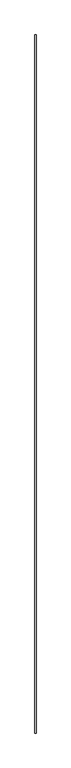
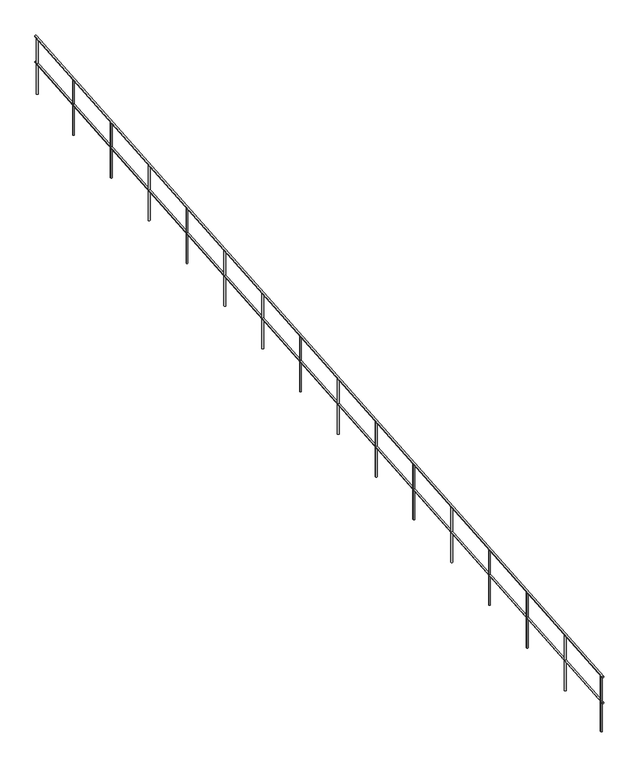
"""IFC4 building model written with IfcOpenShell, lengths in millimetres: railing geometry."""

from ifc_helpers import new_model, si_unit, frame, origin, place, context, project, spatial, ellipse_curve, source, transform, mapped, element, save
from ifc_brep_helpers import plane_surface, cylinder_surface, advanced_brep


def railing_917cd56d(model_context):
    return source(origin(), model_context, "Body", "AdvancedBrep", [
        advanced_brep(
        [(-7531.0, 39498.9598199, -615.0519932), (-7501.0, 39498.9598199, -615.0519932), (-7531.0, 57498.9598198, 884.9480068), (-7501.0, 57498.9598198, 884.9480068)],
        [
            (0, 1, ellipse_curve(frame((-7516.0, 39498.9598199, -615.0519932), z_axis=(0.0, -1.0, 0.0), x_axis=(0.0, 0.0, -0.9999999999999999)), 15.0519932, 15.0)),
            (1, 0, ellipse_curve(frame((-7516.0, 39498.9598199, -615.0519932), z_axis=(0.0, -1.0, 0.0), x_axis=(0.0, 0.0, -0.9999999999999999)), 15.0519932, 15.0)),
            (2, 3, ellipse_curve(frame((-7516.0, 57498.9598198, 884.9480068), z_axis=(0.0, 1.0, 0.0), x_axis=(0.0, 0.0, -0.9999999999999999)), 15.0519932, 15.0)),
            (3, 2, ellipse_curve(frame((-7516.0, 57498.9598198, 884.9480068), z_axis=(0.0, 1.0, 0.0), x_axis=(0.0, 0.0, -0.9999999999999999)), 15.0519932, 15.0)),
            (0, 2),
            (3, 1),
        ],
        [
            plane_surface(frame((-7516.0, 39498.9598199, -600.0), z_axis=(0.0, -1.0, 0.0), x_axis=(0.0, 0.0, 1.0))),
            plane_surface(frame((-7516.0, 57498.9598198, 900.0), z_axis=(0.0, 1.0, 0.0), x_axis=(0.0, 0.0, 1.0))),
            cylinder_surface(frame((-7516.0, 39500.2055021, -614.9481864), z_axis=(0.0, -0.9965457582448797, -0.08304547985373997), x_axis=(1.0, 0.0, 0.0)), 15.0),
        ],
        [
            (0, [[1, 2]]),
            (1, [[3, 4]]),
            (2, [[-1, 5, -4, 6]]),
            (2, [[-2, -6, -3, -5]]),
        ],
    ),
        advanced_brep(
        [(-7531.0, 39498.9598199, -115.0519932), (-7501.0, 39498.9598199, -115.0519932), (-7531.0, 57498.9598198, 1384.9480068), (-7501.0, 57498.9598198, 1384.9480068)],
        [
            (0, 1, ellipse_curve(frame((-7516.0, 39498.9598199, -115.0519932), z_axis=(0.0, -1.0, 0.0), x_axis=(0.0, 0.0, -0.9999999999999999)), 15.0519932, 15.0)),
            (1, 0, ellipse_curve(frame((-7516.0, 39498.9598199, -115.0519932), z_axis=(0.0, -1.0, 0.0), x_axis=(0.0, 0.0, -0.9999999999999999)), 15.0519932, 15.0)),
            (2, 3, ellipse_curve(frame((-7516.0, 57498.9598198, 1384.9480068), z_axis=(0.0, 1.0, 0.0), x_axis=(0.0, 0.0, -0.9999999999999999)), 15.0519932, 15.0)),
            (3, 2, ellipse_curve(frame((-7516.0, 57498.9598198, 1384.9480068), z_axis=(0.0, 1.0, 0.0), x_axis=(0.0, 0.0, -0.9999999999999999)), 15.0519932, 15.0)),
            (0, 2),
            (3, 1),
        ],
        [
            plane_surface(frame((-7516.0, 39498.9598199, -100.0), z_axis=(0.0, -1.0, 0.0), x_axis=(0.0, 0.0, 1.0))),
            plane_surface(frame((-7516.0, 57498.9598198, 1400.0), z_axis=(0.0, 1.0, 0.0), x_axis=(0.0, 0.0, 1.0))),
            cylinder_surface(frame((-7516.0, 39500.2055021, -114.9481864), z_axis=(0.0, -0.9965457582448797, -0.08304547985373997), x_axis=(1.0, 0.0, 0.0)), 15.0),
        ],
        [
            (0, [[1, 2]]),
            (1, [[3, 4]]),
            (2, [[-1, 5, -4, 6]]),
            (2, [[-2, -6, -3, -5]]),
        ],
    ),
        advanced_brep(
        [(-7501.0, 56298.9598199, 1269.8960136), (-7501.0, 56298.9598199, 200.0), (-7531.0, 56298.9598199, 200.0), (-7531.0, 56298.9598199, 1269.8960136)],
        [
            (0, 1),
            (1, 2, ellipse_curve(frame((-7516.0, 56298.9598199, 200.0), z_axis=(0.0, -0.08304547985373996, 0.9965457582448797), x_axis=(0.0, 0.9965457582448798, 0.08304547985373881)), 15.0519932, 15.0)),
            (2, 3),
            (3, 0, ellipse_curve(frame((-7516.0, 56298.9598199, 1269.8960136), z_axis=(0.0, 0.083045479853741, -0.9965457582448796), x_axis=(0.0, 0.9965457582448797, 0.08304547985374044)), 15.0519932, 15.0)),
            (0, 3, ellipse_curve(frame((-7516.0, 56298.9598199, 1269.8960136), z_axis=(0.0, 0.083045479853741, -0.9965457582448796), x_axis=(0.0, 0.9965457582448797, 0.08304547985374044)), 15.0519932, 15.0)),
            (2, 1, ellipse_curve(frame((-7516.0, 56298.9598199, 200.0), z_axis=(0.0, -0.08304547985373996, 0.9965457582448797), x_axis=(0.0, 0.9965457582448798, 0.08304547985373881)), 15.0519932, 15.0)),
        ],
        [
            cylinder_surface(frame((-7516.0, 56298.9598199, 100.0), z_axis=(0.0, 0.0, 1.0), x_axis=(-1.0, 0.0, 0.0)), 15.0),
            plane_surface(frame((-7541.0, 56323.9598199, 1271.9793469), z_axis=(0.0, -0.083045479853741, 0.9965457582448796), x_axis=(1.0, 0.0, 0.0))),
            plane_surface(frame((-7541.0, 56273.9598199, 197.9166667), z_axis=(0.0, 0.08304547985373996, -0.9965457582448797), x_axis=(1.0, 0.0, 0.0))),
        ],
        [
            (0, [[1, 2, 3, 4]]),
            (0, [[-1, 5, -3, 6]]),
            (1, [[-4, -5]]),
            (2, [[-2, -6]]),
        ],
    ),
        advanced_brep(
        [(-7501.0, 55098.9598199, 1169.8960136), (-7501.0, 55098.9598199, 100.0), (-7531.0, 55098.9598199, 100.0), (-7531.0, 55098.9598199, 1169.8960136)],
        [
            (0, 1),
            (1, 2, ellipse_curve(frame((-7516.0, 55098.9598199, 100.0), z_axis=(0.0, -0.08304547985373996, 0.9965457582448797), x_axis=(0.0, 0.9965457582448798, 0.08304547985373881)), 15.0519932, 15.0)),
            (2, 3),
            (3, 0, ellipse_curve(frame((-7516.0, 55098.9598199, 1169.8960136), z_axis=(0.0, 0.083045479853741, -0.9965457582448796), x_axis=(0.0, 0.9965457582448797, 0.08304547985374044)), 15.0519932, 15.0)),
            (0, 3, ellipse_curve(frame((-7516.0, 55098.9598199, 1169.8960136), z_axis=(0.0, 0.083045479853741, -0.9965457582448796), x_axis=(0.0, 0.9965457582448797, 0.08304547985374044)), 15.0519932, 15.0)),
            (2, 1, ellipse_curve(frame((-7516.0, 55098.9598199, 100.0), z_axis=(0.0, -0.08304547985373996, 0.9965457582448797), x_axis=(0.0, 0.9965457582448798, 0.08304547985373881)), 15.0519932, 15.0)),
        ],
        [
            cylinder_surface(frame((-7516.0, 55098.9598199, 0.0), z_axis=(0.0, 0.0, 1.0), x_axis=(-1.0, 0.0, 0.0)), 15.0),
            plane_surface(frame((-7541.0, 55123.9598199, 1171.9793469), z_axis=(0.0, -0.083045479853741, 0.9965457582448796), x_axis=(1.0, 0.0, 0.0))),
            plane_surface(frame((-7541.0, 55073.9598199, 97.9166667), z_axis=(0.0, 0.08304547985373996, -0.9965457582448797), x_axis=(1.0, 0.0, 0.0))),
        ],
        [
            (0, [[1, 2, 3, 4]]),
            (0, [[-1, 5, -3, 6]]),
            (1, [[-4, -5]]),
            (2, [[-2, -6]]),
        ],
    ),
        advanced_brep(
        [(-7501.0, 53898.9598199, 1069.8960136), (-7501.0, 53898.9598199, 0.0), (-7531.0, 53898.9598199, 0.0), (-7531.0, 53898.9598199, 1069.8960136)],
        [
            (0, 1),
            (1, 2, ellipse_curve(frame((-7516.0, 53898.9598199, 0.0), z_axis=(0.0, -0.08304547985373996, 0.9965457582448797), x_axis=(0.0, 0.9965457582448798, 0.08304547985373881)), 15.0519932, 15.0)),
            (2, 3),
            (3, 0, ellipse_curve(frame((-7516.0, 53898.9598199, 1069.8960136), z_axis=(0.0, 0.083045479853741, -0.9965457582448796), x_axis=(0.0, 0.9965457582448797, 0.08304547985374044)), 15.0519932, 15.0)),
            (0, 3, ellipse_curve(frame((-7516.0, 53898.9598199, 1069.8960136), z_axis=(0.0, 0.083045479853741, -0.9965457582448796), x_axis=(0.0, 0.9965457582448797, 0.08304547985374044)), 15.0519932, 15.0)),
            (2, 1, ellipse_curve(frame((-7516.0, 53898.9598199, 0.0), z_axis=(0.0, -0.08304547985373996, 0.9965457582448797), x_axis=(0.0, 0.9965457582448798, 0.08304547985373881)), 15.0519932, 15.0)),
        ],
        [
            cylinder_surface(frame((-7516.0, 53898.9598199, -100.0), z_axis=(0.0, 0.0, 1.0), x_axis=(-1.0, 0.0, 0.0)), 15.0),
            plane_surface(frame((-7541.0, 53923.9598199, 1071.9793469), z_axis=(0.0, -0.083045479853741, 0.9965457582448796), x_axis=(1.0, 0.0, 0.0))),
            plane_surface(frame((-7541.0, 53873.9598199, -2.0833333), z_axis=(0.0, 0.08304547985373996, -0.9965457582448797), x_axis=(1.0, 0.0, 0.0))),
        ],
        [
            (0, [[1, 2, 3, 4]]),
            (0, [[-1, 5, -3, 6]]),
            (1, [[-4, -5]]),
            (2, [[-2, -6]]),
        ],
    ),
        advanced_brep(
        [(-7501.0, 52698.9598199, 969.8960136), (-7501.0, 52698.9598199, -100.0), (-7531.0, 52698.9598199, -100.0), (-7531.0, 52698.9598199, 969.8960136)],
        [
            (0, 1),
            (1, 2, ellipse_curve(frame((-7516.0, 52698.9598199, -100.0), z_axis=(0.0, -0.08304547985373996, 0.9965457582448797), x_axis=(0.0, 0.9965457582448798, 0.08304547985373881)), 15.0519932, 15.0)),
            (2, 3),
            (3, 0, ellipse_curve(frame((-7516.0, 52698.9598199, 969.8960136), z_axis=(0.0, 0.083045479853741, -0.9965457582448796), x_axis=(0.0, 0.9965457582448797, 0.08304547985374044)), 15.0519932, 15.0)),
            (0, 3, ellipse_curve(frame((-7516.0, 52698.9598199, 969.8960136), z_axis=(0.0, 0.083045479853741, -0.9965457582448796), x_axis=(0.0, 0.9965457582448797, 0.08304547985374044)), 15.0519932, 15.0)),
            (2, 1, ellipse_curve(frame((-7516.0, 52698.9598199, -100.0), z_axis=(0.0, -0.08304547985373996, 0.9965457582448797), x_axis=(0.0, 0.9965457582448798, 0.08304547985373881)), 15.0519932, 15.0)),
        ],
        [
            cylinder_surface(frame((-7516.0, 52698.9598199, -200.0), z_axis=(0.0, 0.0, 1.0), x_axis=(-1.0, 0.0, 0.0)), 15.0),
            plane_surface(frame((-7541.0, 52723.9598199, 971.9793469), z_axis=(0.0, -0.083045479853741, 0.9965457582448796), x_axis=(1.0, 0.0, 0.0))),
            plane_surface(frame((-7541.0, 52673.9598199, -102.0833333), z_axis=(0.0, 0.08304547985373996, -0.9965457582448797), x_axis=(1.0, 0.0, 0.0))),
        ],
        [
            (0, [[1, 2, 3, 4]]),
            (0, [[-1, 5, -3, 6]]),
            (1, [[-4, -5]]),
            (2, [[-2, -6]]),
        ],
    ),
        advanced_brep(
        [(-7501.0, 51498.9598199, 869.8960136), (-7501.0, 51498.9598199, -200.0), (-7531.0, 51498.9598199, -200.0), (-7531.0, 51498.9598199, 869.8960136)],
        [
            (0, 1),
            (1, 2, ellipse_curve(frame((-7516.0, 51498.9598199, -200.0), z_axis=(0.0, -0.08304547985373996, 0.9965457582448797), x_axis=(0.0, 0.9965457582448798, 0.08304547985373881)), 15.0519932, 15.0)),
            (2, 3),
            (3, 0, ellipse_curve(frame((-7516.0, 51498.9598199, 869.8960136), z_axis=(0.0, 0.083045479853741, -0.9965457582448796), x_axis=(0.0, 0.9965457582448797, 0.08304547985374044)), 15.0519932, 15.0)),
            (0, 3, ellipse_curve(frame((-7516.0, 51498.9598199, 869.8960136), z_axis=(0.0, 0.083045479853741, -0.9965457582448796), x_axis=(0.0, 0.9965457582448797, 0.08304547985374044)), 15.0519932, 15.0)),
            (2, 1, ellipse_curve(frame((-7516.0, 51498.9598199, -200.0), z_axis=(0.0, -0.08304547985373996, 0.9965457582448797), x_axis=(0.0, 0.9965457582448798, 0.08304547985373881)), 15.0519932, 15.0)),
        ],
        [
            cylinder_surface(frame((-7516.0, 51498.9598199, -300.0), z_axis=(0.0, 0.0, 1.0), x_axis=(-1.0, 0.0, 0.0)), 15.0),
            plane_surface(frame((-7541.0, 51523.9598199, 871.9793469), z_axis=(0.0, -0.083045479853741, 0.9965457582448796), x_axis=(1.0, 0.0, 0.0))),
            plane_surface(frame((-7541.0, 51473.9598199, -202.0833333), z_axis=(0.0, 0.08304547985373996, -0.9965457582448797), x_axis=(1.0, 0.0, 0.0))),
        ],
        [
            (0, [[1, 2, 3, 4]]),
            (0, [[-1, 5, -3, 6]]),
            (1, [[-4, -5]]),
            (2, [[-2, -6]]),
        ],
    ),
        advanced_brep(
        [(-7501.0, 50298.9598199, 769.8960136), (-7501.0, 50298.9598199, -300.0), (-7531.0, 50298.9598199, -300.0), (-7531.0, 50298.9598199, 769.8960136)],
        [
            (0, 1),
            (1, 2, ellipse_curve(frame((-7516.0, 50298.9598199, -300.0), z_axis=(0.0, -0.08304547985373996, 0.9965457582448797), x_axis=(0.0, 0.9965457582448798, 0.08304547985373881)), 15.0519932, 15.0)),
            (2, 3),
            (3, 0, ellipse_curve(frame((-7516.0, 50298.9598199, 769.8960136), z_axis=(0.0, 0.083045479853741, -0.9965457582448796), x_axis=(0.0, 0.9965457582448797, 0.08304547985374044)), 15.0519932, 15.0)),
            (0, 3, ellipse_curve(frame((-7516.0, 50298.9598199, 769.8960136), z_axis=(0.0, 0.083045479853741, -0.9965457582448796), x_axis=(0.0, 0.9965457582448797, 0.08304547985374044)), 15.0519932, 15.0)),
            (2, 1, ellipse_curve(frame((-7516.0, 50298.9598199, -300.0), z_axis=(0.0, -0.08304547985373996, 0.9965457582448797), x_axis=(0.0, 0.9965457582448798, 0.08304547985373881)), 15.0519932, 15.0)),
        ],
        [
            cylinder_surface(frame((-7516.0, 50298.9598199, -400.0), z_axis=(0.0, 0.0, 1.0), x_axis=(-1.0, 0.0, 0.0)), 15.0),
            plane_surface(frame((-7541.0, 50323.9598199, 771.9793469), z_axis=(0.0, -0.083045479853741, 0.9965457582448796), x_axis=(1.0, 0.0, 0.0))),
            plane_surface(frame((-7541.0, 50273.9598199, -302.0833333), z_axis=(0.0, 0.08304547985373996, -0.9965457582448797), x_axis=(1.0, 0.0, 0.0))),
        ],
        [
            (0, [[1, 2, 3, 4]]),
            (0, [[-1, 5, -3, 6]]),
            (1, [[-4, -5]]),
            (2, [[-2, -6]]),
        ],
    ),
        advanced_brep(
        [(-7501.0, 49098.9598199, 669.8960136), (-7501.0, 49098.9598199, -400.0), (-7531.0, 49098.9598199, -400.0), (-7531.0, 49098.9598199, 669.8960136)],
        [
            (0, 1),
            (1, 2, ellipse_curve(frame((-7516.0, 49098.9598199, -400.0), z_axis=(0.0, -0.08304547985373996, 0.9965457582448797), x_axis=(0.0, 0.9965457582448798, 0.08304547985373881)), 15.0519932, 15.0)),
            (2, 3),
            (3, 0, ellipse_curve(frame((-7516.0, 49098.9598199, 669.8960136), z_axis=(0.0, 0.083045479853741, -0.9965457582448796), x_axis=(0.0, 0.9965457582448797, 0.08304547985374044)), 15.0519932, 15.0)),
            (0, 3, ellipse_curve(frame((-7516.0, 49098.9598199, 669.8960136), z_axis=(0.0, 0.083045479853741, -0.9965457582448796), x_axis=(0.0, 0.9965457582448797, 0.08304547985374044)), 15.0519932, 15.0)),
            (2, 1, ellipse_curve(frame((-7516.0, 49098.9598199, -400.0), z_axis=(0.0, -0.08304547985373996, 0.9965457582448797), x_axis=(0.0, 0.9965457582448798, 0.08304547985373881)), 15.0519932, 15.0)),
        ],
        [
            cylinder_surface(frame((-7516.0, 49098.9598199, -500.0), z_axis=(0.0, 0.0, 1.0), x_axis=(-1.0, 0.0, 0.0)), 15.0),
            plane_surface(frame((-7541.0, 49123.9598199, 671.9793469), z_axis=(0.0, -0.083045479853741, 0.9965457582448796), x_axis=(1.0, 0.0, 0.0))),
            plane_surface(frame((-7541.0, 49073.9598199, -402.0833333), z_axis=(0.0, 0.08304547985373996, -0.9965457582448797), x_axis=(1.0, 0.0, 0.0))),
        ],
        [
            (0, [[1, 2, 3, 4]]),
            (0, [[-1, 5, -3, 6]]),
            (1, [[-4, -5]]),
            (2, [[-2, -6]]),
        ],
    ),
        advanced_brep(
        [(-7501.0, 47898.9598199, 569.8960136), (-7501.0, 47898.9598199, -500.0), (-7531.0, 47898.9598199, -500.0), (-7531.0, 47898.9598199, 569.8960136)],
        [
            (0, 1),
            (1, 2, ellipse_curve(frame((-7516.0, 47898.9598199, -500.0), z_axis=(0.0, -0.08304547985373996, 0.9965457582448797), x_axis=(0.0, 0.9965457582448798, 0.08304547985373881)), 15.0519932, 15.0)),
            (2, 3),
            (3, 0, ellipse_curve(frame((-7516.0, 47898.9598199, 569.8960136), z_axis=(0.0, 0.083045479853741, -0.9965457582448796), x_axis=(0.0, 0.9965457582448797, 0.08304547985374044)), 15.0519932, 15.0)),
            (0, 3, ellipse_curve(frame((-7516.0, 47898.9598199, 569.8960136), z_axis=(0.0, 0.083045479853741, -0.9965457582448796), x_axis=(0.0, 0.9965457582448797, 0.08304547985374044)), 15.0519932, 15.0)),
            (2, 1, ellipse_curve(frame((-7516.0, 47898.9598199, -500.0), z_axis=(0.0, -0.08304547985373996, 0.9965457582448797), x_axis=(0.0, 0.9965457582448798, 0.08304547985373881)), 15.0519932, 15.0)),
        ],
        [
            cylinder_surface(frame((-7516.0, 47898.9598199, -600.0), z_axis=(0.0, 0.0, 1.0), x_axis=(-1.0, 0.0, 0.0)), 15.0),
            plane_surface(frame((-7541.0, 47923.9598199, 571.9793469), z_axis=(0.0, -0.083045479853741, 0.9965457582448796), x_axis=(1.0, 0.0, 0.0))),
            plane_surface(frame((-7541.0, 47873.9598199, -502.0833333), z_axis=(0.0, 0.08304547985373996, -0.9965457582448797), x_axis=(1.0, 0.0, 0.0))),
        ],
        [
            (0, [[1, 2, 3, 4]]),
            (0, [[-1, 5, -3, 6]]),
            (1, [[-4, -5]]),
            (2, [[-2, -6]]),
        ],
    ),
        advanced_brep(
        [(-7501.0, 46698.9598199, 469.8960136), (-7501.0, 46698.9598199, -600.0), (-7531.0, 46698.9598199, -600.0), (-7531.0, 46698.9598199, 469.8960136)],
        [
            (0, 1),
            (1, 2, ellipse_curve(frame((-7516.0, 46698.9598199, -600.0), z_axis=(0.0, -0.08304547985373996, 0.9965457582448797), x_axis=(0.0, 0.9965457582448798, 0.08304547985373881)), 15.0519932, 15.0)),
            (2, 3),
            (3, 0, ellipse_curve(frame((-7516.0, 46698.9598199, 469.8960136), z_axis=(0.0, 0.083045479853741, -0.9965457582448796), x_axis=(0.0, 0.9965457582448797, 0.08304547985374044)), 15.0519932, 15.0)),
            (0, 3, ellipse_curve(frame((-7516.0, 46698.9598199, 469.8960136), z_axis=(0.0, 0.083045479853741, -0.9965457582448796), x_axis=(0.0, 0.9965457582448797, 0.08304547985374044)), 15.0519932, 15.0)),
            (2, 1, ellipse_curve(frame((-7516.0, 46698.9598199, -600.0), z_axis=(0.0, -0.08304547985373996, 0.9965457582448797), x_axis=(0.0, 0.9965457582448798, 0.08304547985373881)), 15.0519932, 15.0)),
        ],
        [
            cylinder_surface(frame((-7516.0, 46698.9598199, -700.0), z_axis=(0.0, 0.0, 1.0), x_axis=(-1.0, 0.0, 0.0)), 15.0),
            plane_surface(frame((-7541.0, 46723.9598199, 471.9793469), z_axis=(0.0, -0.083045479853741, 0.9965457582448796), x_axis=(1.0, 0.0, 0.0))),
            plane_surface(frame((-7541.0, 46673.9598199, -602.0833333), z_axis=(0.0, 0.08304547985373996, -0.9965457582448797), x_axis=(1.0, 0.0, 0.0))),
        ],
        [
            (0, [[1, 2, 3, 4]]),
            (0, [[-1, 5, -3, 6]]),
            (1, [[-4, -5]]),
            (2, [[-2, -6]]),
        ],
    ),
        advanced_brep(
        [(-7501.0, 45498.9598199, 369.8960136), (-7501.0, 45498.9598199, -700.0), (-7531.0, 45498.9598199, -700.0), (-7531.0, 45498.9598199, 369.8960136)],
        [
            (0, 1),
            (1, 2, ellipse_curve(frame((-7516.0, 45498.9598199, -700.0), z_axis=(0.0, -0.08304547985373996, 0.9965457582448797), x_axis=(0.0, 0.9965457582448798, 0.08304547985373881)), 15.0519932, 15.0)),
            (2, 3),
            (3, 0, ellipse_curve(frame((-7516.0, 45498.9598199, 369.8960136), z_axis=(0.0, 0.083045479853741, -0.9965457582448796), x_axis=(0.0, 0.9965457582448797, 0.08304547985374044)), 15.0519932, 15.0)),
            (0, 3, ellipse_curve(frame((-7516.0, 45498.9598199, 369.8960136), z_axis=(0.0, 0.083045479853741, -0.9965457582448796), x_axis=(0.0, 0.9965457582448797, 0.08304547985374044)), 15.0519932, 15.0)),
            (2, 1, ellipse_curve(frame((-7516.0, 45498.9598199, -700.0), z_axis=(0.0, -0.08304547985373996, 0.9965457582448797), x_axis=(0.0, 0.9965457582448798, 0.08304547985373881)), 15.0519932, 15.0)),
        ],
        [
            cylinder_surface(frame((-7516.0, 45498.9598199, -800.0), z_axis=(0.0, 0.0, 1.0), x_axis=(-1.0, 0.0, 0.0)), 15.0),
            plane_surface(frame((-7541.0, 45523.9598199, 371.9793469), z_axis=(0.0, -0.083045479853741, 0.9965457582448796), x_axis=(1.0, 0.0, 0.0))),
            plane_surface(frame((-7541.0, 45473.9598199, -702.0833333), z_axis=(0.0, 0.08304547985373996, -0.9965457582448797), x_axis=(1.0, 0.0, 0.0))),
        ],
        [
            (0, [[1, 2, 3, 4]]),
            (0, [[-1, 5, -3, 6]]),
            (1, [[-4, -5]]),
            (2, [[-2, -6]]),
        ],
    ),
        advanced_brep(
        [(-7501.0, 44298.9598199, 269.8960136), (-7501.0, 44298.9598199, -800.0), (-7531.0, 44298.9598199, -800.0), (-7531.0, 44298.9598199, 269.8960136)],
        [
            (0, 1),
            (1, 2, ellipse_curve(frame((-7516.0, 44298.9598199, -800.0), z_axis=(0.0, -0.08304547985373996, 0.9965457582448797), x_axis=(0.0, 0.9965457582448798, 0.08304547985373881)), 15.0519932, 15.0)),
            (2, 3),
            (3, 0, ellipse_curve(frame((-7516.0, 44298.9598199, 269.8960136), z_axis=(0.0, 0.083045479853741, -0.9965457582448796), x_axis=(0.0, 0.9965457582448797, 0.08304547985374044)), 15.0519932, 15.0)),
            (0, 3, ellipse_curve(frame((-7516.0, 44298.9598199, 269.8960136), z_axis=(0.0, 0.083045479853741, -0.9965457582448796), x_axis=(0.0, 0.9965457582448797, 0.08304547985374044)), 15.0519932, 15.0)),
            (2, 1, ellipse_curve(frame((-7516.0, 44298.9598199, -800.0), z_axis=(0.0, -0.08304547985373996, 0.9965457582448797), x_axis=(0.0, 0.9965457582448798, 0.08304547985373881)), 15.0519932, 15.0)),
        ],
        [
            cylinder_surface(frame((-7516.0, 44298.9598199, -900.0), z_axis=(0.0, 0.0, 1.0), x_axis=(-1.0, 0.0, 0.0)), 15.0),
            plane_surface(frame((-7541.0, 44323.9598199, 271.9793469), z_axis=(0.0, -0.083045479853741, 0.9965457582448796), x_axis=(1.0, 0.0, 0.0))),
            plane_surface(frame((-7541.0, 44273.9598199, -802.0833333), z_axis=(0.0, 0.08304547985373996, -0.9965457582448797), x_axis=(1.0, 0.0, 0.0))),
        ],
        [
            (0, [[1, 2, 3, 4]]),
            (0, [[-1, 5, -3, 6]]),
            (1, [[-4, -5]]),
            (2, [[-2, -6]]),
        ],
    ),
        advanced_brep(
        [(-7501.0, 43098.9598199, 169.8960136), (-7501.0, 43098.9598199, -900.0), (-7531.0, 43098.9598199, -900.0), (-7531.0, 43098.9598199, 169.8960136)],
        [
            (0, 1),
            (1, 2, ellipse_curve(frame((-7516.0, 43098.9598199, -900.0), z_axis=(0.0, -0.08304547985373996, 0.9965457582448797), x_axis=(0.0, 0.9965457582448798, 0.08304547985373881)), 15.0519932, 15.0)),
            (2, 3),
            (3, 0, ellipse_curve(frame((-7516.0, 43098.9598199, 169.8960136), z_axis=(0.0, 0.083045479853741, -0.9965457582448796), x_axis=(0.0, 0.9965457582448797, 0.08304547985374044)), 15.0519932, 15.0)),
            (0, 3, ellipse_curve(frame((-7516.0, 43098.9598199, 169.8960136), z_axis=(0.0, 0.083045479853741, -0.9965457582448796), x_axis=(0.0, 0.9965457582448797, 0.08304547985374044)), 15.0519932, 15.0)),
            (2, 1, ellipse_curve(frame((-7516.0, 43098.9598199, -900.0), z_axis=(0.0, -0.08304547985373996, 0.9965457582448797), x_axis=(0.0, 0.9965457582448798, 0.08304547985373881)), 15.0519932, 15.0)),
        ],
        [
            cylinder_surface(frame((-7516.0, 43098.9598199, -1000.0), z_axis=(0.0, 0.0, 1.0), x_axis=(-1.0, 0.0, 0.0)), 15.0),
            plane_surface(frame((-7541.0, 43123.9598199, 171.9793469), z_axis=(0.0, -0.083045479853741, 0.9965457582448796), x_axis=(1.0, 0.0, 0.0))),
            plane_surface(frame((-7541.0, 43073.9598199, -902.0833333), z_axis=(0.0, 0.08304547985373996, -0.9965457582448797), x_axis=(1.0, 0.0, 0.0))),
        ],
        [
            (0, [[1, 2, 3, 4]]),
            (0, [[-1, 5, -3, 6]]),
            (1, [[-4, -5]]),
            (2, [[-2, -6]]),
        ],
    ),
        advanced_brep(
        [(-7501.0, 41898.9598199, 69.8960136), (-7501.0, 41898.9598199, -1000.0), (-7531.0, 41898.9598199, -1000.0), (-7531.0, 41898.9598199, 69.8960136)],
        [
            (0, 1),
            (1, 2, ellipse_curve(frame((-7516.0, 41898.9598199, -1000.0), z_axis=(0.0, -0.08304547985373996, 0.9965457582448797), x_axis=(0.0, 0.9965457582448798, 0.08304547985373881)), 15.0519932, 15.0)),
            (2, 3),
            (3, 0, ellipse_curve(frame((-7516.0, 41898.9598199, 69.8960136), z_axis=(0.0, 0.083045479853741, -0.9965457582448796), x_axis=(0.0, 0.9965457582448797, 0.08304547985374044)), 15.0519932, 15.0)),
            (0, 3, ellipse_curve(frame((-7516.0, 41898.9598199, 69.8960136), z_axis=(0.0, 0.083045479853741, -0.9965457582448796), x_axis=(0.0, 0.9965457582448797, 0.08304547985374044)), 15.0519932, 15.0)),
            (2, 1, ellipse_curve(frame((-7516.0, 41898.9598199, -1000.0), z_axis=(0.0, -0.08304547985373996, 0.9965457582448797), x_axis=(0.0, 0.9965457582448798, 0.08304547985373881)), 15.0519932, 15.0)),
        ],
        [
            cylinder_surface(frame((-7516.0, 41898.9598199, -1100.0), z_axis=(0.0, 0.0, 1.0), x_axis=(-1.0, 0.0, 0.0)), 15.0),
            plane_surface(frame((-7541.0, 41923.9598199, 71.9793469), z_axis=(0.0, -0.083045479853741, 0.9965457582448796), x_axis=(1.0, 0.0, 0.0))),
            plane_surface(frame((-7541.0, 41873.9598199, -1002.0833333), z_axis=(0.0, 0.08304547985373996, -0.9965457582448797), x_axis=(1.0, 0.0, 0.0))),
        ],
        [
            (0, [[1, 2, 3, 4]]),
            (0, [[-1, 5, -3, 6]]),
            (1, [[-4, -5]]),
            (2, [[-2, -6]]),
        ],
    ),
        advanced_brep(
        [(-7501.0, 40698.9598199, -30.1039864), (-7501.0, 40698.9598199, -1100.0), (-7531.0, 40698.9598199, -1100.0), (-7531.0, 40698.9598199, -30.1039864)],
        [
            (0, 1),
            (1, 2, ellipse_curve(frame((-7516.0, 40698.9598199, -1100.0), z_axis=(0.0, -0.08304547985373996, 0.9965457582448797), x_axis=(0.0, 0.9965457582448798, 0.08304547985373881)), 15.0519932, 15.0)),
            (2, 3),
            (3, 0, ellipse_curve(frame((-7516.0, 40698.9598199, -30.1039864), z_axis=(0.0, 0.083045479853741, -0.9965457582448796), x_axis=(0.0, 0.9965457582448797, 0.08304547985374044)), 15.0519932, 15.0)),
            (0, 3, ellipse_curve(frame((-7516.0, 40698.9598199, -30.1039864), z_axis=(0.0, 0.083045479853741, -0.9965457582448796), x_axis=(0.0, 0.9965457582448797, 0.08304547985374044)), 15.0519932, 15.0)),
            (2, 1, ellipse_curve(frame((-7516.0, 40698.9598199, -1100.0), z_axis=(0.0, -0.08304547985373996, 0.9965457582448797), x_axis=(0.0, 0.9965457582448798, 0.08304547985373881)), 15.0519932, 15.0)),
        ],
        [
            cylinder_surface(frame((-7516.0, 40698.9598199, -1200.0), z_axis=(0.0, 0.0, 1.0), x_axis=(-1.0, 0.0, 0.0)), 15.0),
            plane_surface(frame((-7541.0, 40723.9598199, -28.0206531), z_axis=(0.0, -0.083045479853741, 0.9965457582448796), x_axis=(1.0, 0.0, 0.0))),
            plane_surface(frame((-7541.0, 40673.9598199, -1102.0833333), z_axis=(0.0, 0.08304547985373996, -0.9965457582448797), x_axis=(1.0, 0.0, 0.0))),
        ],
        [
            (0, [[1, 2, 3, 4]]),
            (0, [[-1, 5, -3, 6]]),
            (1, [[-4, -5]]),
            (2, [[-2, -6]]),
        ],
    ),
        advanced_brep(
        [(-7501.0, 57448.9598198, 1365.7293469), (-7501.0, 57448.9598198, 295.8333333), (-7531.0, 57448.9598198, 295.8333333), (-7531.0, 57448.9598198, 1365.7293469)],
        [
            (0, 1),
            (1, 2, ellipse_curve(frame((-7516.0, 57448.9598198, 295.8333333), z_axis=(0.0, -0.08304547985373996, 0.9965457582448797), x_axis=(0.0, 0.9965457582448798, 0.08304547985373881)), 15.0519932, 15.0)),
            (2, 3),
            (3, 0, ellipse_curve(frame((-7516.0, 57448.9598198, 1365.7293469), z_axis=(0.0, 0.083045479853741, -0.9965457582448796), x_axis=(0.0, 0.9965457582448797, 0.08304547985374044)), 15.0519932, 15.0)),
            (0, 3, ellipse_curve(frame((-7516.0, 57448.9598198, 1365.7293469), z_axis=(0.0, 0.083045479853741, -0.9965457582448796), x_axis=(0.0, 0.9965457582448797, 0.08304547985374044)), 15.0519932, 15.0)),
            (2, 1, ellipse_curve(frame((-7516.0, 57448.9598198, 295.8333333), z_axis=(0.0, -0.08304547985373996, 0.9965457582448797), x_axis=(0.0, 0.9965457582448798, 0.08304547985373881)), 15.0519932, 15.0)),
        ],
        [
            cylinder_surface(frame((-7516.0, 57448.9598198, 195.8333333), z_axis=(0.0, 0.0, 1.0), x_axis=(-1.0, 0.0, 0.0)), 15.0),
            plane_surface(frame((-7541.0, 57473.9598198, 1367.8126802), z_axis=(0.0, -0.083045479853741, 0.9965457582448796), x_axis=(1.0, 0.0, 0.0))),
            plane_surface(frame((-7541.0, 57423.9598198, 293.75), z_axis=(0.0, 0.08304547985373996, -0.9965457582448797), x_axis=(1.0, 0.0, 0.0))),
        ],
        [
            (0, [[1, 2, 3, 4]]),
            (0, [[-1, 5, -3, 6]]),
            (1, [[-4, -5]]),
            (2, [[-2, -6]]),
        ],
    ),
        advanced_brep(
        [(-7501.0, 39548.9598199, -125.9373198), (-7501.0, 39548.9598199, -1195.8333333), (-7531.0, 39548.9598199, -1195.8333333), (-7531.0, 39548.9598199, -125.9373198)],
        [
            (0, 1),
            (1, 2, ellipse_curve(frame((-7516.0, 39548.9598199, -1195.8333333), z_axis=(0.0, -0.08304547985373996, 0.9965457582448797), x_axis=(0.0, 0.9965457582448798, 0.08304547985373881)), 15.0519932, 15.0)),
            (2, 3),
            (3, 0, ellipse_curve(frame((-7516.0, 39548.9598199, -125.9373198), z_axis=(0.0, 0.083045479853741, -0.9965457582448796), x_axis=(0.0, 0.9965457582448797, 0.08304547985374044)), 15.0519932, 15.0)),
            (0, 3, ellipse_curve(frame((-7516.0, 39548.9598199, -125.9373198), z_axis=(0.0, 0.083045479853741, -0.9965457582448796), x_axis=(0.0, 0.9965457582448797, 0.08304547985374044)), 15.0519932, 15.0)),
            (2, 1, ellipse_curve(frame((-7516.0, 39548.9598199, -1195.8333333), z_axis=(0.0, -0.08304547985373996, 0.9965457582448797), x_axis=(0.0, 0.9965457582448798, 0.08304547985373881)), 15.0519932, 15.0)),
        ],
        [
            cylinder_surface(frame((-7516.0, 39548.9598199, -1295.8333333), z_axis=(0.0, 0.0, 1.0), x_axis=(-1.0, 0.0, 0.0)), 15.0),
            plane_surface(frame((-7541.0, 39573.9598199, -123.8539864), z_axis=(0.0, -0.083045479853741, 0.9965457582448796), x_axis=(1.0, 0.0, 0.0))),
            plane_surface(frame((-7541.0, 39523.9598199, -1197.9166667), z_axis=(0.0, 0.08304547985373996, -0.9965457582448797), x_axis=(1.0, 0.0, 0.0))),
        ],
        [
            (0, [[1, 2, 3, 4]]),
            (0, [[-1, 5, -3, 6]]),
            (1, [[-4, -5]]),
            (2, [[-2, -6]]),
        ],
    ),
    ])


if __name__ == "__main__":
    model = new_model("IFC4")
    model_context = context("Model", 3, world=origin())
    ifc_project = project(units=[si_unit("LENGTHUNIT", "METRE", prefix="MILLI")], contexts=[model_context])
    site = spatial("IfcSite", under=ifc_project)
    building = spatial("IfcBuilding", under=site)
    placement = place(None, origin())
    railing_shape = railing_917cd56d(model_context)
    element("IfcRailing", 1, at=placement, inside=building, context=model_context, shape_type="MappedRepresentation", body=[
        mapped(railing_shape, transform((0.0, 0.0, 0.0), x_axis=(1.0, 0.0, 0.0), y_axis=(0.0, 1.0, 0.0), z_axis=(0.0, 0.0, 1.0))),
    ])
    save(model, "model.ifc")
